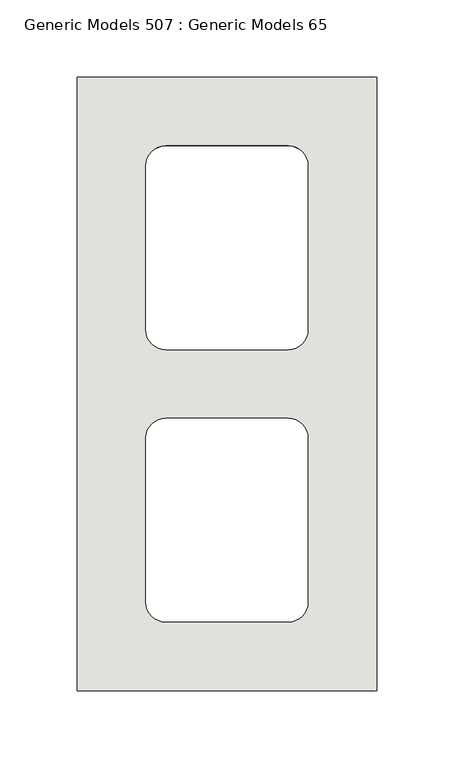
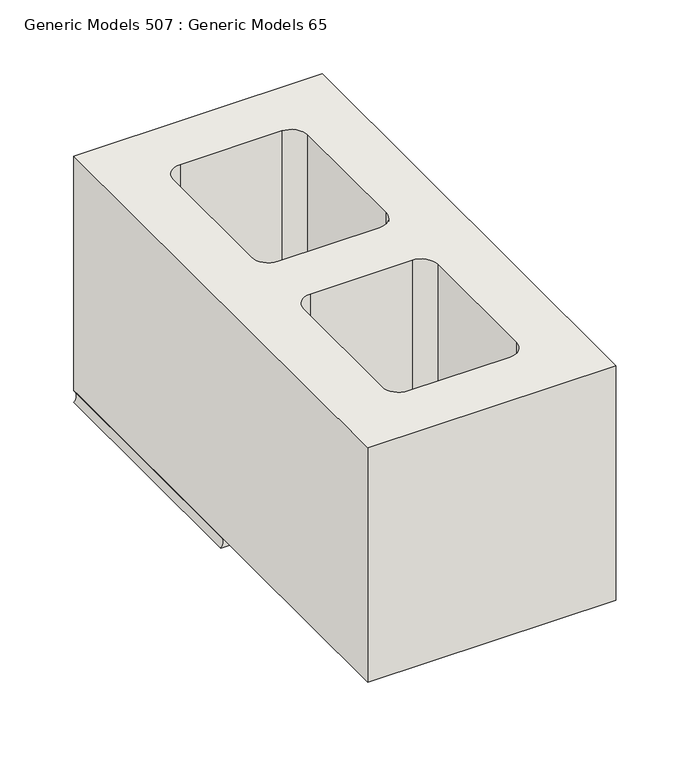
"""IFC4 building model written with IfcOpenShell, lengths in millimetres: wall geometry, Generic Models 507 : Generic Models 65."""

from ifc_helpers import new_model, si_unit, point, frame, frame_2d, origin, place, context, project, spatial, polyline, circle_curve, trimmed, segment, composite_curve, outline, extrude, source, transform, mapped, element, save
from ifc_brep_helpers import plane_surface, revolved_surface, advanced_brep


def generic_models_507_generic_models_65_b6502902(model_context):
    return source(origin(), model_context, "Body", "SolidModel", [
        advanced_brep(
        [(428979.0125, 503.2375, 822.325), (428785.3375, 503.2375, 822.325), (428785.3375, 503.2375, 812.8), (428979.0125, 503.2375, 812.8), (428979.0125, 701.675, 822.325), (428979.0125, 701.675, 812.8), (428785.3375, 701.675, 812.8), (428785.3375, 701.675, 822.325), (428934.5625, 538.1625, 822.325), (428921.8625, 525.4625, 822.325), (428842.4875, 525.4625, 822.325), (428829.7875, 538.1625, 822.325), (428829.7875, 644.525, 822.325), (428842.4875, 657.225, 822.325), (428921.8625, 657.225, 822.325), (428934.5625, 644.525, 822.325), (428921.8625, 525.4625, 812.8), (428934.5625, 538.1625, 812.8), (428842.4875, 525.4625, 812.8), (428829.7875, 538.1625, 812.8), (428829.7875, 644.525, 812.8), (428842.4875, 657.225, 812.8), (428921.8625, 657.225, 812.8), (428934.5625, 644.525, 812.8)],
        [
            (0, 1),
            (1, 2, circle_curve(frame((428780.4545028, 503.2375, 817.5625), z_axis=(0.0, 1.0, 0.0), x_axis=(1.0, 0.0, 0.0)), 6.8209287)),
            (2, 3),
            (3, 0, circle_curve(frame((428983.8954972, 503.2375, 817.5625), z_axis=(0.0, 1.0, 0.0), x_axis=(-1.0, 0.0, 0.0)), 6.8209287)),
            (4, 5, circle_curve(frame((428983.8954972, 701.675, 817.5625), z_axis=(0.0, -1.0, 0.0), x_axis=(-1.0, 0.0, 0.0)), 6.8209287)),
            (5, 6),
            (6, 7, circle_curve(frame((428780.4545028, 701.675, 817.5625), z_axis=(0.0, -1.0, 0.0), x_axis=(1.0, 0.0, 0.0)), 6.8209287)),
            (7, 4),
            (0, 4),
            (7, 1),
            (8, 9, circle_curve(frame((428921.8625, 538.1625, 822.325), z_axis=(0.0, 0.0, -1.0), x_axis=(-1.0, 0.0, 0.0)), 12.7)),
            (9, 10),
            (10, 11, circle_curve(frame((428842.4875, 538.1625, 822.325), z_axis=(0.0, 0.0, -1.0), x_axis=(-1.0, 0.0, 0.0)), 12.7)),
            (11, 12),
            (12, 13, circle_curve(frame((428842.4875, 644.525, 822.325), z_axis=(0.0, 0.0, -1.0), x_axis=(-1.0, 0.0, 0.0)), 12.7)),
            (13, 14),
            (14, 15, circle_curve(frame((428921.8625, 644.525, 822.325), z_axis=(0.0, 0.0, -1.0), x_axis=(-1.0, 0.0, 0.0)), 12.7)),
            (15, 8),
            (16, 9),
            (8, 17),
            (17, 16, circle_curve(frame((428921.8625, 538.1625, 812.8), z_axis=(0.0, 0.0, -1.0), x_axis=(-1.0, 0.0, 0.0)), 12.7)),
            (16, 18),
            (18, 10),
            (18, 19, circle_curve(frame((428842.4875, 538.1625, 812.8), z_axis=(0.0, 0.0, -1.0), x_axis=(-1.0, 0.0, 0.0)), 12.7)),
            (19, 11),
            (19, 20),
            (20, 12),
            (20, 21, circle_curve(frame((428842.4875, 644.525, 812.8), z_axis=(0.0, 0.0, -1.0), x_axis=(-1.0, 0.0, 0.0)), 12.7)),
            (21, 13),
            (21, 22),
            (22, 14),
            (22, 23, circle_curve(frame((428921.8625, 644.525, 812.8), z_axis=(0.0, 0.0, -1.0), x_axis=(-1.0, 0.0, 0.0)), 12.7)),
            (23, 15),
            (23, 17),
            (6, 2),
            (5, 3),
        ],
        [
            plane_surface(frame((428882.175, 503.2375, 822.721875), z_axis=(0.0, -1.0, 0.0), x_axis=(0.0, 0.0, 1.0))),
            plane_surface(frame((428882.175, 701.675, 822.721875), z_axis=(0.0, 1.0, 0.0), x_axis=(0.0, 0.0, 1.0))),
            plane_surface(frame((428979.0125, 503.2375, 822.325), z_axis=(0.0, 0.0, 1.0), x_axis=(0.0, 1.0, 0.0))),
            revolved_surface(polyline([(428909.1625, 538.1625, 822.325), (428909.1625, 538.1625, 812.8)]), (428921.8625, 538.1625, 1006.475), (0.0, 0.0, 1.0)),
            plane_surface(frame((428842.4875, 525.4625, 1006.475), z_axis=(0.0, 1.0, 0.0), x_axis=(0.0, 0.0, -1.0))),
            revolved_surface(polyline([(428829.7875, 538.1625, 822.325), (428829.7875, 538.1625, 812.8)]), (428842.4875, 538.1625, 1006.475), (0.0, 0.0, 1.0)),
            plane_surface(frame((428829.7875, 644.525, 1006.475), z_axis=(1.0, 0.0, 0.0), x_axis=(0.0, 0.0, -1.0))),
            revolved_surface(polyline([(428829.7875, 644.525, 822.325), (428829.7875, 644.525, 812.8)]), (428842.4875, 644.525, 1006.475), (0.0, 0.0, 1.0)),
            plane_surface(frame((428921.8625, 657.225, 1006.475), z_axis=(0.0, -1.0, 0.0), x_axis=(0.0, 0.0, -1.0))),
            revolved_surface(polyline([(428909.1625, 644.525, 822.325), (428909.1625, 644.525, 812.8)]), (428921.8625, 644.525, 1006.475), (0.0, 0.0, 1.0)),
            plane_surface(frame((428934.5625, 538.1625, 1006.475), z_axis=(-1.0, 0.0, 0.0), x_axis=(0.0, 0.0, -1.0))),
            revolved_surface(polyline([(428787.2754315, 701.675, 817.5625), (428787.2754315, 503.2375, 817.5625)]), (428780.4545028, 503.2375, 817.5625), (0.0, 1.0, 0.0)),
            plane_surface(frame((428785.3375, 503.2375, 812.8), z_axis=(0.0, 0.0, -1.0), x_axis=(0.0, 1.0, 0.0))),
            revolved_surface(polyline([(428977.07456850004, 701.675, 817.5625), (428977.07456850004, 503.2375, 817.5625)]), (428983.8954972, 503.2375, 817.5625), (0.0, 1.0, 0.0)),
        ],
        [
            (0, [[1, 2, 3, 4]]),
            (1, [[5, 6, 7, 8]]),
            (2, [[-1, 9, -8, 10], [11, 12, 13, 14, 15, 16, 17, 18]]),
            (3, [[19, -11, 20, 21]]),
            (4, [[-19, 22, 23, -12]]),
            (5, [[-23, 24, 25, -13]]),
            (6, [[-25, 26, 27, -14]]),
            (7, [[-27, 28, 29, -15]]),
            (8, [[-29, 30, 31, -16]]),
            (9, [[-31, 32, 33, -17]]),
            (10, [[-33, 34, -20, -18]]),
            (11, [[-2, -10, -7, 35]]),
            (12, [[-3, -35, -6, 36], [-21, -34, -32, -30, -28, -26, -24, -22]]),
            (13, [[-4, -36, -5, -9]]),
        ],
    ),
        extrude(outline(polyline([(428979.0125, 304.8), (428785.3375, 304.8), (428785.3375, 701.675), (428979.0125, 701.675), (428979.0125, 304.8)]), holes=[composite_curve([segment(polyline([(428934.5625, 538.1625), (428934.5625, 644.525)]), True, "CONTINUOUS"), segment(trimmed(circle_curve(frame_2d((428921.8625, 644.525)), 12.7), [point((428934.5625, 644.525))], [point((428921.8625, 657.225))], True, "CARTESIAN"), True, "CONTINUOUS"), segment(polyline([(428921.8625, 657.225), (428842.4875, 657.225)]), True, "CONTINUOUS"), segment(trimmed(circle_curve(frame_2d((428842.4875, 644.525)), 12.7), [point((428842.4875, 657.225))], [point((428829.7875, 644.525))], True, "CARTESIAN"), True, "CONTINUOUS"), segment(polyline([(428829.7875, 644.525), (428829.7875, 538.1625)]), True, "CONTINUOUS"), segment(trimmed(circle_curve(frame_2d((428842.4875, 538.1625)), 12.7), [point((428829.7875, 538.1625))], [point((428842.4875, 525.4625))], True, "CARTESIAN"), True, "CONTINUOUS"), segment(polyline([(428842.4875, 525.4625), (428921.8625, 525.4625)]), True, "CONTINUOUS"), segment(trimmed(circle_curve(frame_2d((428921.8625, 538.1625)), 12.7), [point((428921.8625, 525.4625))], [point((428934.5625, 538.1625))], True, "CARTESIAN"), True, "CONTINUOUS")], self_intersect=False), composite_curve([segment(polyline([(428829.7875, 468.3125), (428829.7875, 361.95)]), True, "CONTINUOUS"), segment(trimmed(circle_curve(frame_2d((428842.4875, 361.95)), 12.7), [point((428829.7875, 361.95))], [point((428842.4875, 349.25))], True, "CARTESIAN"), True, "CONTINUOUS"), segment(polyline([(428842.4875, 349.25), (428921.8625, 349.25)]), True, "CONTINUOUS"), segment(trimmed(circle_curve(frame_2d((428921.8625, 361.95)), 12.7), [point((428921.8625, 349.25))], [point((428934.5625, 361.95))], True, "CARTESIAN"), True, "CONTINUOUS"), segment(polyline([(428934.5625, 361.95), (428934.5625, 468.3125)]), True, "CONTINUOUS"), segment(trimmed(circle_curve(frame_2d((428921.8625, 468.3125)), 12.7), [point((428934.5625, 468.3125))], [point((428921.8625, 481.0125))], True, "CARTESIAN"), True, "CONTINUOUS"), segment(polyline([(428921.8625, 481.0125), (428842.4875, 481.0125)]), True, "CONTINUOUS"), segment(trimmed(circle_curve(frame_2d((428842.4875, 468.3125)), 12.7), [point((428842.4875, 481.0125))], [point((428829.7875, 468.3125))], True, "CARTESIAN"), True, "CONTINUOUS")], self_intersect=False)]), frame((0.0, 0.0, 822.325), z_axis=(0.0, 0.0, 1.0), x_axis=(1.0, 0.0, 0.0)), (0.0, 0.0, 1.0), 193.675),
    ])


if __name__ == "__main__":
    model = new_model("IFC4")
    model_context = context("Model", 3, world=origin())
    ifc_project = project(units=[si_unit("LENGTHUNIT", "METRE", prefix="MILLI")], contexts=[model_context])
    site = spatial("IfcSite", under=ifc_project)
    building = spatial("IfcBuilding", under=site)
    placement = place(None, origin())
    generic_models_507_generic_models_65_shape = generic_models_507_generic_models_65_b6502902(model_context)
    element("IfcWall", 1, ObjectType="Generic Models 507 : Generic Models 65", at=placement, inside=building, context=model_context, shape_type="MappedRepresentation", body=[
        mapped(generic_models_507_generic_models_65_shape, transform((0.0, 0.0, 0.0), x_axis=(1.0, 0.0, 0.0), y_axis=(0.0, 1.0, 0.0), z_axis=(0.0, 0.0, 1.0))),
    ])
    save(model, "model.ifc")

# Revit data of these elements
# Element 1 (IfcWall, "Generic Models 507 : Generic Models 65")
#   Materials on its faces: "CMU (SEE 'WALL TAG' FOR SIZE)", "MORTAR JOINT"
# Materials
#   "CMU (SEE 'WALL TAG' FOR SIZE)": class "Masonry", colour RGB 203 203 199, transparency 0, Description = "Concrete masonry units", Cost = 0
#   "MORTAR JOINT": class "Generic", colour RGB 120 120 120, transparency 0, Cost = 0
